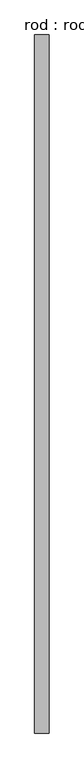
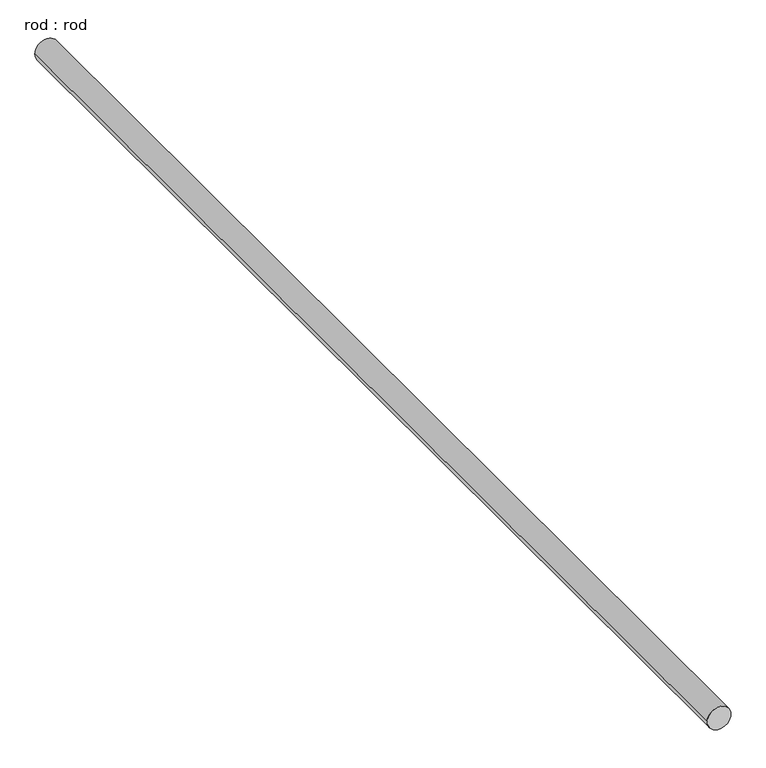
"""IFC4 building model written with IfcOpenShell, lengths in millimetres: proxy geometry, rod : rod."""

from ifc_helpers import new_model, si_unit, point, frame, frame_2d, origin, place, context, project, spatial, circle_curve, trimmed, segment, composite_curve, outline, extrude, source, transform, mapped, element, save


def rod_rod_b1f3397e(model_context):
    return source(origin(), model_context, "Body", "SweptSolid", [
        extrude(outline(composite_curve([segment(trimmed(circle_curve(frame_2d((0.0108462, 0.0)), 200.0), [point((0.0108462, 200.0))], [point((0.0108462, -200.0))], False, "CARTESIAN"), True, "CONTINUOUS"), segment(trimmed(circle_curve(frame_2d((0.0108462, 0.0)), 200.0), [point((0.0108462, -200.0))], [point((0.0108462, 200.0))], False, "CARTESIAN"), True, "CONTINUOUS")], self_intersect=False)), frame((0.0, -5737.6285275, 0.0), z_axis=(0.0, 1.0, 0.0), x_axis=(0.0, 0.0, 1.0)), (0.0, 0.0, 1.0), 19660.7142857),
    ])


if __name__ == "__main__":
    model = new_model("IFC4")
    model_context = context("Model", 3, world=origin())
    ifc_project = project(units=[si_unit("LENGTHUNIT", "METRE", prefix="MILLI")], contexts=[model_context])
    site = spatial("IfcSite", under=ifc_project)
    building = spatial("IfcBuilding", under=site)
    placement = place(None, origin())
    rod_rod_shape = rod_rod_b1f3397e(model_context)
    element("IfcBuildingElementProxy", 1, Name="rod : rod", ObjectType="rod : rod", at=placement, inside=building, context=model_context, shape_type="MappedRepresentation", body=[
        mapped(rod_rod_shape, transform((0.0, 0.0, 0.0), x_axis=(1.0, 0.0, 0.0), y_axis=(0.0, 1.0, 0.0), z_axis=(0.0, 0.0, 1.0))),
    ])
    save(model, "model.ifc")

# Revit data of these elements
# Type "rod : rod"
#   Default Elevation = 0
